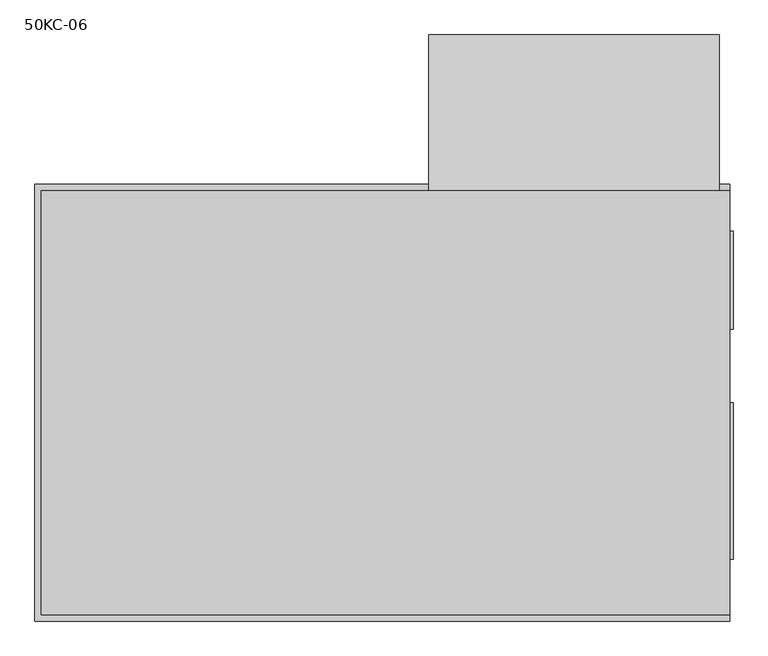
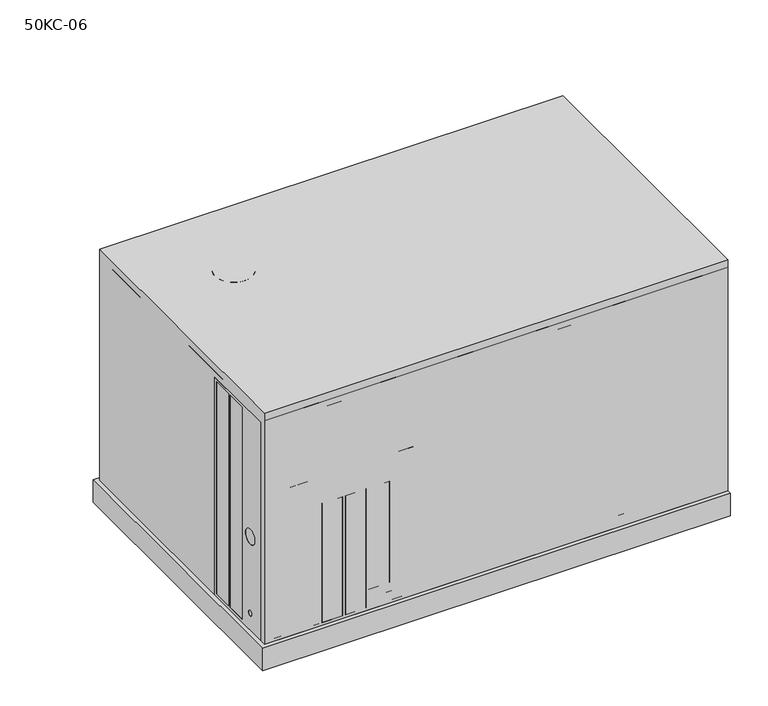
"""IFC4 building model written with IfcOpenShell, lengths in millimetres: proxy geometry, AHU-Rooftop-Carrier-Cooling_&_Elec_Heating-3-5_ton : 50KC-06."""

import ifcopenshell
import ifcopenshell.guid

model = None  # the IFC model being written
_history = None  # IfcOwnerHistory: only IFC2X3 demands one
_inside = {}  # id of a spatial element -> (the spatial element, [elements in it])
_under = {}  # id of a project, library or spatial element -> (it, [spatial elements below it])
_declared = {}  # id of a project -> (the project, [libraries it declares])
_typed = {}  # id of a type object -> (the type object, [elements of that type])
_made_of = {}  # id of a material, layer set ... -> (it, [elements and type objects made of it])


def new_model(schema):
    """Start an empty IFC model of exactly this schema.

    Asked for "IFC4X3", IfcOpenShell would pick the latest addendum, in which some entities
    have other attributes; the version numbers below select the first issue.
    IFC2X3 requires an IfcOwnerHistory on every rooted entity: one is made here for all.
    """
    global model, _history
    if schema == "IFC4X3":
        model = ifcopenshell.file(schema_version=(4, 3, 0, 0))
    else:
        model = ifcopenshell.file(schema=schema)
    _inside.clear()
    _under.clear()
    _declared.clear()
    _typed.clear()
    _made_of.clear()
    _history = None
    if model.schema == "IFC2X3":
        org = make("IfcOrganization", Name="unknown")
        user = make(
            "IfcPersonAndOrganization",
            ThePerson=make("IfcPerson", FamilyName="unknown"),
            TheOrganization=org,
        )
        app = make(
            "IfcApplication",
            ApplicationDeveloper=org,
            Version="unknown",
            ApplicationFullName="unknown",
            ApplicationIdentifier="unknown",
        )
        _history = make(
            "IfcOwnerHistory",
            OwningUser=user,
            OwningApplication=app,
            ChangeAction="ADDED",
            CreationDate=0,
        )
    return model


def make(cls, **values):
    """One entity of the class cls with the attributes given. An attribute that is None is left unset."""
    return model.create_entity(
        cls, **{name: value for name, value in values.items() if value is not None}
    )


def rooted(cls, **values):
    """An entity with a GlobalId (a new one), such as an element, a storey or a relation."""
    return make(cls, GlobalId=ifcopenshell.guid.new(), OwnerHistory=_history, **values)


def si_unit(unit_type, name, prefix=None):
    """IfcSIUnit, for example si_unit("LENGTHUNIT", "METRE", prefix="MILLI")."""
    return make("IfcSIUnit", UnitType=unit_type, Prefix=prefix, Name=name)


def assignment(units):
    """IfcUnitAssignment: the units of a project."""
    return None if units is None else make("IfcUnitAssignment", Units=units)


def point(xyz):
    """IfcCartesianPoint."""
    return None if xyz is None else make("IfcCartesianPoint", Coordinates=xyz)


def direction(xyz):
    """IfcDirection."""
    return None if xyz is None else make("IfcDirection", DirectionRatios=xyz)


def frame(location, z_axis=None, x_axis=None):
    """IfcAxis2Placement3D, a coordinate frame: its origin and axes. An axis left out is left unset."""
    return make(
        "IfcAxis2Placement3D",
        Location=point(location),
        Axis=direction(z_axis),
        RefDirection=direction(x_axis),
    )


def frame_2d(location, x_axis=None):
    """IfcAxis2Placement2D, a coordinate frame in the plane: its origin and x axis."""
    return make(
        "IfcAxis2Placement2D", Location=point(location), RefDirection=direction(x_axis)
    )


def origin():
    """The frame at (0, 0, 0) with its axes left unset."""
    return frame((0.0, 0.0, 0.0))


def origin_with_axes():
    """The frame at (0, 0, 0) with the z axis (0, 0, 1) and the x axis (1, 0, 0) written out."""
    return frame((0.0, 0.0, 0.0), z_axis=(0.0, 0.0, 1.0), x_axis=(1.0, 0.0, 0.0))


def place(relative_to, where):
    """IfcLocalPlacement: puts the frame where relative to a parent placement (None: the world)."""
    return make(
        "IfcLocalPlacement", PlacementRelTo=relative_to, RelativePlacement=where
    )


def context(
    kind, dimensions, precision=None, world=None, true_north=None, identifier=None
):
    """IfcGeometricRepresentationContext, for example the 3D "Model" context."""
    return make(
        "IfcGeometricRepresentationContext",
        ContextIdentifier=identifier,
        ContextType=kind,
        CoordinateSpaceDimension=dimensions,
        Precision=precision,
        WorldCoordinateSystem=world,
        TrueNorth=true_north,
    )


def project(units=None, contexts=None):
    """IfcProject with its units and contexts."""
    return rooted(
        "IfcProject",
        Name="project",
        RepresentationContexts=contexts,
        UnitsInContext=assignment(units),
    )


def spatial(cls, under=None, at=None, **own):
    """A site, building, storey or space (cls), placed at a placement, below another one or the project."""
    s = rooted(cls, ObjectPlacement=at, **own)
    if under is not None:
        _under.setdefault(under.id(), (under, []))[1].append(s)
    return s


def polyline(points):
    """IfcPolyline through the points."""
    return make("IfcPolyline", Points=[point(p) for p in points])


def circle_curve(where, radius):
    """IfcCircle in the frame where."""
    return make("IfcCircle", Position=where, Radius=radius)


def trimmed(basis, trim1, trim2, sense, master):
    """IfcTrimmedCurve: the piece of a basis curve between two trims."""
    return make(
        "IfcTrimmedCurve",
        BasisCurve=basis,
        Trim1=trim1,
        Trim2=trim2,
        SenseAgreement=sense,
        MasterRepresentation=master,
    )


def segment(curve, same_sense, transition):
    """IfcCompositeCurveSegment."""
    return make(
        "IfcCompositeCurveSegment",
        Transition=transition,
        SameSense=same_sense,
        ParentCurve=curve,
    )


def composite_curve(segments, self_intersect=None):
    """IfcCompositeCurve: segments joined end to end."""
    return make("IfcCompositeCurve", Segments=segments, SelfIntersect=self_intersect)


def outline(outer, holes=None, kind="AREA"):
    """IfcArbitraryClosedProfileDef: a profile drawn as a closed curve; with holes, ...WithVoids."""
    if holes is None:
        return make("IfcArbitraryClosedProfileDef", ProfileType=kind, OuterCurve=outer)
    return make(
        "IfcArbitraryProfileDefWithVoids",
        ProfileType=kind,
        OuterCurve=outer,
        InnerCurves=holes,
    )


def extrude(swept, where, along, depth):
    """IfcExtrudedAreaSolid: the profile swept, set in the frame where, extruded along a direction by depth."""
    return make(
        "IfcExtrudedAreaSolid",
        SweptArea=swept,
        Position=where,
        ExtrudedDirection=direction(along),
        Depth=depth,
    )


def faces_of(points, faces, orient=None, outer=None):
    """IfcFace entities. A face is a list of loops; a loop is a list of indices into points, from 0.

    orient and outer hold one flag for each loop. By default every Orientation is true, the
    first loop of a face is its IfcFaceOuterBound and the others are IfcFaceBound.
    """
    made = []
    for i, loops in enumerate(faces):
        bounds = []
        for j, loop in enumerate(loops):
            is_outer = j == 0 if outer is None else outer[i][j]
            bounds.append(
                make(
                    "IfcFaceOuterBound" if is_outer else "IfcFaceBound",
                    Bound=make("IfcPolyLoop", Polygon=[points[k] for k in loop]),
                    Orientation=True if orient is None else orient[i][j],
                )
            )
        made.append(make("IfcFace", Bounds=bounds))
    return made


def faceted_brep(points, faces, orient=None, outer=None, voids=None):
    """IfcFacetedBrep: a solid bounded by flat faces; with voids (closed shells), ...WithVoids."""
    shared = [point(p) for p in points]
    hull = make("IfcClosedShell", CfsFaces=faces_of(shared, faces, orient, outer))
    if voids is None:
        return make("IfcFacetedBrep", Outer=hull)
    return make(
        "IfcFacetedBrepWithVoids",
        Outer=hull,
        Voids=[
            make(cls, CfsFaces=faces_of(shared, fs, o, b)) for cls, fs, o, b in voids
        ],
    )


def shape(context_of_items, identifier, shape_type, items):
    """IfcShapeRepresentation: the items that make up one representation, for example the "Body"."""
    return make(
        "IfcShapeRepresentation",
        ContextOfItems=context_of_items,
        RepresentationIdentifier=identifier,
        RepresentationType=shape_type,
        Items=items,
    )


def source(mapping_origin, context_of_items, identifier, shape_type, items):
    """IfcRepresentationMap: a shape defined once, which mapped items show again and again."""
    return make(
        "IfcRepresentationMap",
        MappingOrigin=mapping_origin,
        MappedRepresentation=shape(context_of_items, identifier, shape_type, items),
    )


def transform(
    local_origin,
    x_axis=None,
    y_axis=None,
    z_axis=None,
    scale=None,
    scale2=None,
    scale3=None,
    uniform=True,
):
    """IfcCartesianTransformationOperator3D, or its non-uniform kind. x_axis, y_axis, z_axis: its Axis1, 2, 3."""
    if uniform:
        return make(
            "IfcCartesianTransformationOperator3D",
            Axis1=direction(x_axis),
            Axis2=direction(y_axis),
            LocalOrigin=point(local_origin),
            Scale=scale,
            Axis3=direction(z_axis),
        )
    return make(
        "IfcCartesianTransformationOperator3DnonUniform",
        Axis1=direction(x_axis),
        Axis2=direction(y_axis),
        LocalOrigin=point(local_origin),
        Scale=scale,
        Axis3=direction(z_axis),
        Scale2=scale2,
        Scale3=scale3,
    )


def mapped(mapping_source, mapping_target):
    """IfcMappedItem: shows the shape of a source again, moved by a transform."""
    return make(
        "IfcMappedItem", MappingSource=mapping_source, MappingTarget=mapping_target
    )


def made_of(thing, what):
    """Note that an element or type object is made of a material, layer set ...; save() writes the relation."""
    if what is not None:
        _made_of.setdefault(what.id(), (what, []))[1].append(thing)
    return thing


def element(
    cls,
    number,
    at=None,
    inside=None,
    cuts=None,
    type_object=None,
    material=None,
    context=None,
    identifier="Body",
    shape_type=None,
    held_by="IfcProductDefinitionShape",
    body=None,
    shapes=None,
    **own,
):
    """One element of the class cls, such as IfcWall. Its Tag is "e" and its number.

    at: its placement. inside: the storey or other place that contains it. cuts: it is an
    opening in that element (IfcRelVoidsElement). A single representation is given by context,
    identifier, shape_type and body (its items); several are given by shapes. held_by: the class
    of the entity that holds the representations. save() writes the other relations.
    """
    e = rooted(cls, Tag="e%d" % number, ObjectPlacement=at, **own)
    if body is not None:
        shapes = [shape(context, identifier, shape_type, body)]
    if shapes is not None:
        e.Representation = make(held_by, Representations=shapes)
    if inside is not None:
        _inside.setdefault(inside.id(), (inside, []))[1].append(e)
    if cuts is not None:
        rooted(
            "IfcRelVoidsElement", RelatingBuildingElement=cuts, RelatedOpeningElement=e
        )
    if type_object is not None:
        _typed.setdefault(type_object.id(), (type_object, []))[1].append(e)
    return made_of(e, material)


def aggregate(whole, parts):
    """IfcRelAggregates: a whole, such as a stair, and the parts it consists of."""
    return rooted("IfcRelAggregates", RelatingObject=whole, RelatedObjects=parts)


def save(model, path):
    """Write the relations noted so far, then the file.

    IfcRelAggregates (storeys below a building ...), IfcRelContainedInSpatialStructure (elements
    in a storey), IfcRelDefinesByType, IfcRelAssociatesMaterial and IfcRelDeclares: one each for
    every whole, place, type object, material and project.
    """
    for whole, parts in _under.values():
        aggregate(whole, parts)
    for where, things in _inside.values():
        rooted(
            "IfcRelContainedInSpatialStructure",
            RelatedElements=things,
            RelatingStructure=where,
        )
    for kind, things in _typed.values():
        rooted("IfcRelDefinesByType", RelatedObjects=things, RelatingType=kind)
    for what, things in _made_of.values():
        rooted("IfcRelAssociatesMaterial", RelatedObjects=things, RelatingMaterial=what)
    for by, libraries in _declared.values():
        rooted("IfcRelDeclares", RelatingContext=by, RelatedDefinitions=libraries)
    model.write(path)


def plane_surface(at):
    """IfcPlane: the flat surface through the origin of the frame at, square to its z axis."""
    return make("IfcPlane", Position=at)


def cylinder_surface(at, radius):
    """IfcCylindricalSurface: all points at the distance radius from the z axis of the frame at."""
    return make("IfcCylindricalSurface", Position=at, Radius=radius)


def revolved_surface(curve, axis_point, axis_direction):
    """IfcSurfaceOfRevolution: the curve turned about the line through axis_point along axis_direction."""
    return make(
        "IfcSurfaceOfRevolution",
        SweptCurve=make("IfcArbitraryOpenProfileDef", ProfileType="CURVE", Curve=curve),
        AxisPosition=make("IfcAxis1Placement", Location=point(axis_point), Axis=direction(axis_direction)),
    )


def advanced_brep(points, edges, surfaces, faces):
    """IfcAdvancedBrep: a solid bounded by faces that lie on surfaces and meet in shared edges.

    An edge is (start, end): straight between two places in points (the first is 0);
    or (start, end, curve); or (start, end, curve, False) where it runs against its curve.
    A face is (place in surfaces, loops), or (place, loops, False) where it looks against
    its surface's normal. A loop lists edges by number (the first is 1), with a minus sign
    where the edge is run from its end to its start. The first loop is the outer one.
    """
    corners = [point(p) for p in points]
    vertices = [make("IfcVertexPoint", VertexGeometry=c) for c in corners]
    made = []
    for start, end, *more in edges:
        made.append(
            make(
                "IfcEdgeCurve",
                EdgeStart=vertices[start],
                EdgeEnd=vertices[end],
                EdgeGeometry=more[0] if more else make("IfcPolyline", Points=[corners[start], corners[end]]),
                SameSense=more[1] if len(more) > 1 else True,
            )
        )
    hull = []
    for where, loops, *sense in faces:
        bounds = []
        for j, loop in enumerate(loops):
            ring = [make("IfcOrientedEdge", EdgeElement=made[abs(k) - 1], Orientation=k > 0) for k in loop]
            bounds.append(
                make(
                    "IfcFaceOuterBound" if j == 0 else "IfcFaceBound",
                    Bound=make("IfcEdgeLoop", EdgeList=ring),
                    Orientation=True,
                )
            )
        hull.append(make("IfcAdvancedFace", Bounds=bounds, FaceSurface=surfaces[where], SameSense=sense[0] if sense else True))
    return make("IfcAdvancedBrep", Outer=make("IfcClosedShell", CfsFaces=hull))


def proxy_50kc_06_755dc8fb(model_context):
    return source(origin(), model_context, "Body", "SolidModel", [
        extrude(outline(polyline([(-547.6875, 1025.525), (-228.6, 1025.525), (-228.6, 95.25), (-547.6875, 95.25), (-547.6875, 1025.525)]), holes=[polyline([(-323.85, 1012.825), (-323.85, 107.95), (-241.3, 107.95), (-241.3, 1012.825), (-323.85, 1012.825)]), polyline([(-419.1, 1012.825), (-419.1, 107.95), (-336.55, 107.95), (-336.55, 1012.825), (-419.1, 1012.825)]), composite_curve([segment(trimmed(circle_curve(frame_2d((-476.25, 495.3)), 31.75), [point((-508.0, 495.3))], [point((-444.5, 495.3))], True, "CARTESIAN"), True, "CONTINUOUS"), segment(trimmed(circle_curve(frame_2d((-476.25, 495.3)), 31.75), [point((-444.5, 495.3))], [point((-508.0, 495.3))], True, "CARTESIAN"), True, "CONTINUOUS")], self_intersect=False), composite_curve([segment(trimmed(circle_curve(frame_2d((-476.25, 168.275)), 11.1125), [point((-487.3625, 168.275))], [point((-465.1375, 168.275))], True, "CARTESIAN"), True, "CONTINUOUS"), segment(trimmed(circle_curve(frame_2d((-476.25, 168.275)), 11.1125), [point((-465.1375, 168.275))], [point((-487.3625, 168.275))], True, "CARTESIAN"), True, "CONTINUOUS")], self_intersect=False)]), frame((-927.1, 0.0, 0.0), z_axis=(1.0, 0.0, 0.0), x_axis=(0.0, 1.0, 0.0)), (0.0, 0.0, 1.0), 3.175),
        advanced_brep(
        [(941.3875, 573.0875, 1025.525), (-436.5625, 573.0875, 1025.525), (-436.5625, 534.9875, 1025.525), (-885.825, 534.9875, 1025.525), (-885.825, -215.9, 1025.525), (-923.925, -215.9, 1025.525), (-923.925, -573.0875, 1025.525), (941.3875, -573.0875, 1025.525), (-883.285, 532.4475, 1025.525), (-436.5625, 532.4475, 1025.525), (-436.5625, -215.9, 1025.525), (-883.285, -215.9, 1025.525), (941.3875, 573.0875, 95.25), (941.3875, -573.0875, 95.25), (-923.925, -573.0875, 95.25), (-923.925, -215.9, 95.25), (-885.825, -215.9, 95.25), (-885.825, 534.9875, 95.25), (-436.5625, 534.9875, 95.25), (-436.5625, 573.0875, 95.25), (-883.285, 532.4475, 95.25), (-883.285, -215.9, 95.25), (-436.5625, -215.9, 95.25), (-436.5625, 532.4475, 95.25), (-923.925, -508.0, 495.3), (-923.925, -444.5, 495.3), (-923.925, -487.3625, 168.275), (-923.925, -465.1375, 168.275), (941.3875, 88.9, 194.1909375), (941.3875, 88.9, 161.4090625), (919.1625, 88.9, 161.4090625), (919.1625, 88.9, 194.1909375), (-914.4, -508.0, 495.3), (-914.4, -444.5, 495.3), (-914.4, -487.3625, 168.275), (-914.4, -465.1375, 168.275)],
        [
            (0, 1),
            (1, 2),
            (2, 3),
            (3, 4),
            (4, 5),
            (5, 6),
            (6, 7),
            (7, 0),
            (8, 9),
            (9, 10),
            (10, 11),
            (11, 8),
            (12, 13),
            (13, 14),
            (14, 15),
            (15, 16),
            (16, 17),
            (17, 18),
            (18, 19),
            (19, 12),
            (20, 21),
            (21, 22),
            (22, 23),
            (23, 20),
            (0, 12),
            (19, 1),
            (5, 15),
            (14, 6),
            (24, 25, circle_curve(frame((-923.925, -476.25, 495.3), z_axis=(1.0, 0.0, 0.0), x_axis=(0.0, 1.0, 0.0)), 31.75)),
            (25, 24, circle_curve(frame((-923.925, -476.25, 495.3), z_axis=(1.0, 0.0, 0.0), x_axis=(0.0, 1.0, 0.0)), 31.75)),
            (26, 27, circle_curve(frame((-923.925, -476.25, 168.275), z_axis=(1.0, 0.0, 0.0), x_axis=(0.0, 1.0, 0.0)), 11.1125)),
            (27, 26, circle_curve(frame((-923.925, -476.25, 168.275), z_axis=(1.0, 0.0, 0.0), x_axis=(0.0, 1.0, 0.0)), 11.1125)),
            (13, 7),
            (28, 29, circle_curve(frame((941.3875, 88.9, 177.8), z_axis=(-1.0, 0.0, 0.0), x_axis=(0.0, 0.0, 1.0)), 16.3909375)),
            (29, 28, circle_curve(frame((941.3875, 88.9, 177.8), z_axis=(-1.0, 0.0, 0.0), x_axis=(0.0, 0.0, 1.0)), 16.3909375)),
            (18, 2),
            (17, 3),
            (16, 4),
            (30, 31, circle_curve(frame((919.1625, 88.9, 177.8), z_axis=(1.0, 0.0, 0.0), x_axis=(0.0, 0.0, 1.0)), 16.3909375)),
            (31, 30, circle_curve(frame((919.1625, 88.9, 177.8), z_axis=(1.0, 0.0, 0.0), x_axis=(0.0, 0.0, 1.0)), 16.3909375)),
            (30, 29),
            (28, 31),
            (32, 33, circle_curve(frame((-914.4, -476.25, 495.3), z_axis=(-1.0, 0.0, 0.0), x_axis=(0.0, 1.0, 0.0)), 31.75)),
            (33, 32, circle_curve(frame((-914.4, -476.25, 495.3), z_axis=(-1.0, 0.0, 0.0), x_axis=(0.0, 1.0, 0.0)), 31.75)),
            (34, 35, circle_curve(frame((-914.4, -476.25, 168.275), z_axis=(-1.0, 0.0, 0.0), x_axis=(0.0, 1.0, 0.0)), 11.1125)),
            (35, 34, circle_curve(frame((-914.4, -476.25, 168.275), z_axis=(-1.0, 0.0, 0.0), x_axis=(0.0, 1.0, 0.0)), 11.1125)),
            (33, 25),
            (24, 32),
            (35, 27),
            (26, 34),
            (8, 20),
            (23, 9),
            (22, 10),
            (21, 11),
        ],
        [
            plane_surface(frame((-466.3462048, 573.0875, 1025.525), z_axis=(0.0, 0.0, 1.0), x_axis=(-1.0, 0.0, 0.0))),
            plane_surface(frame((-466.3462048, 573.0875, 95.25), z_axis=(0.0, 0.0, -1.0), x_axis=(1.0, 0.0, 0.0))),
            plane_surface(frame((941.3875, 573.0875, 1025.525), z_axis=(0.0, 1.0, 0.0), x_axis=(0.0, 0.0, -1.0))),
            plane_surface(frame((-923.925, -215.9, 1025.525), z_axis=(-1.0, 0.0, 0.0), x_axis=(0.0, 0.0, -1.0))),
            plane_surface(frame((-923.925, -573.0875, 1025.525), z_axis=(0.0, -1.0, 0.0), x_axis=(0.0, 0.0, -1.0))),
            plane_surface(frame((941.3875, -573.0875, 1025.525), z_axis=(1.0, 0.0, 0.0), x_axis=(0.0, 0.0, -1.0))),
            plane_surface(frame((-436.5625, 573.0875, 1025.525), z_axis=(-1.0, 0.0, 0.0), x_axis=(0.0, 0.0, -1.0))),
            plane_surface(frame((-436.5625, 534.9875, 1025.525), z_axis=(0.0, 1.0, 0.0), x_axis=(0.0, 0.0, -1.0))),
            plane_surface(frame((-885.825, 534.9875, 1025.525), z_axis=(-1.0, 0.0, 0.0), x_axis=(0.0, 0.0, -1.0))),
            plane_surface(frame((-885.825, -215.9, 1025.525), z_axis=(0.0, 1.0, 0.0), x_axis=(0.0, 0.0, -1.0))),
            plane_surface(frame((919.1625, 88.9, 177.8), z_axis=(1.0, 0.0, 0.0), x_axis=(0.0, 1.0, 0.0))),
            revolved_surface(polyline([(941.3875, 88.9, 194.19093750000002), (919.1625, 88.9, 194.19093750000002)]), (944.5625, 88.9, 177.8), (1.0, 0.0, 0.0)),
            plane_surface(frame((-914.4, -444.5, 495.3), z_axis=(-1.0, 0.0, 0.0), x_axis=(0.0, 0.0, 1.0))),
            revolved_surface(polyline([(-914.4, -444.5, 495.3), (-923.925, -444.5, 495.3)]), (-927.1, -476.25, 495.3), (1.0, 0.0, 0.0)),
            revolved_surface(polyline([(-914.4, -465.1375, 168.275), (-923.925, -465.1375, 168.275)]), (-927.1, -476.25, 168.275), (1.0, 0.0, 0.0)),
            plane_surface(frame((-883.285, 532.4475, 1025.525), z_axis=(0.0, -1.0, 0.0), x_axis=(0.0, 0.0, -1.0))),
            plane_surface(frame((-436.5625, 532.4475, 1025.525), z_axis=(-1.0, 0.0, 0.0), x_axis=(0.0, 0.0, -1.0))),
            plane_surface(frame((-436.5625, -215.9, 1025.525), z_axis=(0.0, 1.0, 0.0), x_axis=(0.0, 0.0, -1.0))),
            plane_surface(frame((-883.285, -215.9, 1025.525), z_axis=(1.0, 0.0, 0.0), x_axis=(0.0, 0.0, -1.0))),
        ],
        [
            (0, [[1, 2, 3, 4, 5, 6, 7, 8], [9, 10, 11, 12]]),
            (1, [[13, 14, 15, 16, 17, 18, 19, 20], [21, 22, 23, 24]]),
            (2, [[-1, 25, -20, 26]]),
            (3, [[-6, 27, -15, 28], [29, 30], [31, 32]]),
            (4, [[-7, -28, -14, 33]]),
            (5, [[-8, -33, -13, -25], [34, 35]]),
            (6, [[-2, -26, -19, 36]]),
            (7, [[-3, -36, -18, 37]]),
            (8, [[-4, -37, -17, 38]]),
            (9, [[-5, -38, -16, -27]]),
            (10, [[39, 40]]),
            (11, [[-39, 41, -34, 42]]),
            (11, [[-40, -42, -35, -41]]),
            (12, [[43, 44]]),
            (12, [[45, 46]]),
            (13, [[-44, 47, -29, 48]]),
            (13, [[-43, -48, -30, -47]]),
            (14, [[-46, 49, -31, 50]]),
            (14, [[-45, -50, -32, -49]]),
            (15, [[-9, 51, -24, 52]]),
            (16, [[-10, -52, -23, 53]]),
            (17, [[-11, -53, -22, 54]]),
            (18, [[-12, -54, -21, -51]]),
        ],
    ),
        faceted_brep([(-898.525, 573.0875, 1025.525), (-923.925, 573.0875, 1025.525), (-923.925, 547.6875, 1025.525), (-898.525, 547.6875, 1025.525), (-898.525, 573.0875, 95.25), (-898.525, 547.6875, 95.25), (-923.925, 547.6875, 95.25), (-923.925, 573.0875, 95.25)], [[[0, 1, 2, 3]], [[4, 5, 6, 7]], [[1, 0, 4, 7]], [[2, 1, 7, 6]], [[3, 2, 6, 5]], [[0, 3, 5, 4]]]),
        extrude(outline(polyline([(941.3875, 466.725), (954.0875, 466.725), (954.0875, 200.025), (941.3875, 200.025), (941.3875, 466.725)])), frame((0.0, 0.0, 155.575), z_axis=(0.0, 0.0, 1.0), x_axis=(1.0, 0.0, 0.0)), (0.0, 0.0, 1.0), 638.175),
        extrude(outline(polyline([(941.3875, 0.0), (954.0875, 0.0), (954.0875, -425.45), (941.3875, -425.45), (941.3875, 0.0)])), frame((0.0, 0.0, 155.575), z_axis=(0.0, 0.0, 1.0), x_axis=(1.0, 0.0, 0.0)), (0.0, 0.0, 1.0), 288.925),
        extrude(outline(polyline([(944.5625, 576.2625), (944.5625, -576.2625), (-927.1, -576.2625), (-927.1, 576.2625), (944.5625, 576.2625)])), frame((0.0, 0.0, 95.25), z_axis=(0.0, 0.0, 1.0), x_axis=(1.0, 0.0, 0.0)), (0.0, 0.0, 1.0), 987.425),
        extrude(outline(polyline([(-944.5625, 593.725), (944.5625, 593.725), (944.5625, -593.725), (-944.5625, -593.725), (-944.5625, 593.725)])), origin_with_axes(), (0.0, 0.0, 1.0), 95.25),
        extrude(outline(polyline([(21.43125, -576.2625), (-3.96875, -576.2625), (-3.96875, 576.2625), (21.43125, 576.2625), (21.43125, -576.2625)])), frame((0.0, 0.0, 1050.925), z_axis=(0.0, 0.0, 1.0), x_axis=(1.0, 0.0, 0.0)), (0.0, 0.0, 1.0), 12.7),
        extrude(outline(polyline([(1025.525, -411.1625), (95.25, -411.1625), (95.25, 101.6), (1025.525, 101.6), (1025.525, -411.1625)]), holes=[polyline([(177.8, -202.40625), (177.8, -107.15625), (146.05, -107.15625), (146.05, -202.40625), (177.8, -202.40625)])]), frame((0.0, 573.0875, 0.0), z_axis=(0.0, 1.0, 0.0), x_axis=(0.0, 0.0, 1.0)), (0.0, 0.0, 1.0), 3.175),
        extrude(outline(polyline([(915.9875, 573.0875), (127.0, 573.0875), (127.0, 576.2625), (915.9875, 576.2625), (915.9875, 573.0875)])), frame((0.0, 0.0, 546.1), z_axis=(0.0, 0.0, 1.0), x_axis=(1.0, 0.0, 0.0)), (0.0, 0.0, 1.0), 479.425),
        extrude(outline(polyline([(915.9875, 573.0875), (127.0, 573.0875), (127.0, 576.2625), (915.9875, 576.2625), (915.9875, 573.0875)])), frame((0.0, 0.0, 95.25), z_axis=(0.0, 0.0, 1.0), x_axis=(1.0, 0.0, 0.0)), (0.0, 0.0, 1.0), 444.5),
        extrude(outline(polyline([(-923.925, -336.55), (-923.925, -419.1), (-927.1, -419.1), (-927.1, -336.55), (-923.925, -336.55)])), frame((0.0, 0.0, 107.95), z_axis=(0.0, 0.0, 1.0), x_axis=(1.0, 0.0, 0.0)), (0.0, 0.0, 1.0), 904.875),
        extrude(outline(polyline([(-923.925, -241.3), (-923.925, -323.85), (-927.1, -323.85), (-927.1, -241.3), (-923.925, -241.3)])), frame((0.0, 0.0, 107.95), z_axis=(0.0, 0.0, 1.0), x_axis=(1.0, 0.0, 0.0)), (0.0, 0.0, 1.0), 904.875),
        extrude(outline(polyline([(-803.275, -576.2625), (-885.825, -576.2625), (-885.825, -573.0875), (-803.275, -573.0875), (-803.275, -576.2625)])), frame((0.0, 0.0, 107.95), z_axis=(0.0, 0.0, 1.0), x_axis=(1.0, 0.0, 0.0)), (0.0, 0.0, 1.0), 622.3),
        extrude(outline(polyline([(-708.025, -576.2625), (-790.575, -576.2625), (-790.575, -573.0875), (-708.025, -573.0875), (-708.025, -576.2625)])), frame((0.0, 0.0, 107.95), z_axis=(0.0, 0.0, 1.0), x_axis=(1.0, 0.0, 0.0)), (0.0, 0.0, 1.0), 622.3),
        extrude(outline(polyline([(-612.775, -576.2625), (-695.325, -576.2625), (-695.325, -573.0875), (-612.775, -573.0875), (-612.775, -576.2625)])), frame((0.0, 0.0, 107.95), z_axis=(0.0, 0.0, 1.0), x_axis=(1.0, 0.0, 0.0)), (0.0, 0.0, 1.0), 508.0),
        extrude(outline(polyline([(-517.525, -576.2625), (-600.075, -576.2625), (-600.075, -573.0875), (-517.525, -573.0875), (-517.525, -576.2625)])), frame((0.0, 0.0, 107.95), z_axis=(0.0, 0.0, 1.0), x_axis=(1.0, 0.0, 0.0)), (0.0, 0.0, 1.0), 508.0),
        extrude(outline(polyline([(-422.275, -576.2625), (-504.825, -576.2625), (-504.825, -573.0875), (-422.275, -573.0875), (-422.275, -576.2625)])), frame((0.0, 0.0, 184.15), z_axis=(0.0, 0.0, 1.0), x_axis=(1.0, 0.0, 0.0)), (0.0, 0.0, 1.0), 431.8),
        extrude(outline(polyline([(-327.025, -576.2625), (-409.575, -576.2625), (-409.575, -573.0875), (-327.025, -573.0875), (-327.025, -576.2625)])), frame((0.0, 0.0, 107.95), z_axis=(0.0, 0.0, 1.0), x_axis=(1.0, 0.0, 0.0)), (0.0, 0.0, 1.0), 622.3),
        extrude(outline(polyline([(1025.525, 915.9875), (1025.525, 34.13125), (95.25, 34.13125), (95.25, 915.9875), (1025.525, 915.9875)]), holes=[polyline([(177.8, 522.684375), (146.05, 522.684375), (146.05, 427.434375), (177.8, 427.434375), (177.8, 522.684375)])]), frame((0.0, -576.2625, 0.0), z_axis=(0.0, 1.0, 0.0), x_axis=(0.0, 0.0, 1.0)), (0.0, 0.0, 1.0), 3.175),
        extrude(outline(polyline([(1025.525, -16.66875), (1025.525, -898.525), (95.25, -898.525), (95.25, -16.66875), (1025.525, -16.66875)]), holes=[polyline([(177.8, -415.925), (146.05, -415.925), (146.05, -511.175), (177.8, -511.175), (177.8, -415.925)]), polyline([(730.25, -803.275), (107.95, -803.275), (107.95, -885.825), (730.25, -885.825), (730.25, -803.275)]), polyline([(730.25, -708.025), (107.95, -708.025), (107.95, -790.575), (730.25, -790.575), (730.25, -708.025)]), polyline([(615.95, -612.775), (107.95, -612.775), (107.95, -695.325), (615.95, -695.325), (615.95, -612.775)]), polyline([(615.95, -517.525), (107.95, -517.525), (107.95, -600.075), (615.95, -600.075), (615.95, -517.525)]), polyline([(615.95, -422.275), (184.15, -422.275), (184.15, -504.825), (615.95, -504.825), (615.95, -422.275)]), polyline([(730.25, -327.025), (107.95, -327.025), (107.95, -409.575), (730.25, -409.575), (730.25, -327.025)])]), frame((0.0, -576.2625, 0.0), z_axis=(0.0, 1.0, 0.0), x_axis=(0.0, 0.0, 1.0)), (0.0, 0.0, 1.0), 3.175),
        extrude(outline(polyline([(1000.125, 464.451767), (997.9196681, 451.9447085), (947.8914343, 460.7660359), (709.1843069, 119.8569277), (573.0875, 107.95), (573.0875, 539.75), (1000.125, 464.451767)])), frame((127.0, 0.0, 0.0), z_axis=(1.0, 0.0, 0.0), x_axis=(0.0, 1.0, 0.0)), (0.0, 0.0, 1.0), 788.9875),
        advanced_brep(
        [(-584.2, 233.3625, 1082.675), (-660.4, 233.3625, 1082.675), (-508.0, 233.3625, 1082.675), (-660.4, 233.3625, 1079.5), (-508.0, 233.3625, 1079.5), (-863.6, 233.3625, 1050.925), (-304.8, 233.3625, 1050.925), (-584.2, 233.3625, 1050.925)],
        [
            (0, 1),
            (1, 2, circle_curve(frame((-584.2, 233.3625, 1082.675), z_axis=(0.0, 0.0, 1.0), x_axis=(-1.0, 0.0, 0.0)), 76.2)),
            (2, 0),
            (2, 1, circle_curve(frame((-584.2, 233.3625, 1082.675), z_axis=(0.0, 0.0, 1.0), x_axis=(-1.0, 0.0, 0.0)), 76.2)),
            (1, 3),
            (3, 4, circle_curve(frame((-584.2, 233.3625, 1079.5), z_axis=(0.0, 0.0, 1.0), x_axis=(-1.0, 0.0, 0.0)), 76.2)),
            (4, 2),
            (4, 3, circle_curve(frame((-584.2, 233.3625, 1079.5), z_axis=(0.0, 0.0, 1.0), x_axis=(-1.0, 0.0, 0.0)), 76.2)),
            (3, 5),
            (5, 6, circle_curve(frame((-584.2, 233.3625, 1050.925), z_axis=(0.0, 0.0, 1.0), x_axis=(-1.0, 0.0, 0.0)), 279.4)),
            (6, 4),
            (6, 5, circle_curve(frame((-584.2, 233.3625, 1050.925), z_axis=(0.0, 0.0, 1.0), x_axis=(-1.0, 0.0, 0.0)), 279.4)),
            (5, 7),
            (7, 6),
        ],
        [
            plane_surface(frame((-584.2, 233.3625, 1082.675), z_axis=(0.0, 0.0, 1.0), x_axis=(-1.0, 0.0, 0.0))),
            cylinder_surface(frame((-584.2, 233.3625, 1654.166912), z_axis=(0.0, 0.0, 1.0), x_axis=(-1.0, 0.0, 0.0)), 76.2),
            revolved_surface(polyline([(-863.6, 233.3625, 1050.925), (-660.4, 233.3625, 1079.5)]), (-584.2, 233.3625, 1654.166912), (0.0, 0.0, 1.0)),
            plane_surface(frame((-584.2, 233.3625, 1050.925), z_axis=(0.0, 0.0, -1.0), x_axis=(-1.0, 0.0, 0.0))),
        ],
        [
            (0, [[1, 2, 3]]),
            (0, [[-3, 4, -1]]),
            (1, [[-2, 5, 6, 7]]),
            (1, [[-4, -7, 8, -5]]),
            (2, [[-6, 9, 10, 11]]),
            (2, [[-8, -11, 12, -9]]),
            (3, [[-10, 13, 14]]),
            (3, [[-12, -14, -13]]),
        ],
    ),
        extrude(outline(polyline([(944.5625, 576.2625), (944.5625, -576.2625), (-927.1, -576.2625), (-927.1, 576.2625), (944.5625, 576.2625)])), frame((0.0, 0.0, 1025.525), z_axis=(0.0, 0.0, 1.0), x_axis=(1.0, 0.0, 0.0)), (0.0, 0.0, 1.0), 25.4),
        extrude(outline(polyline([(944.5625, 593.725), (944.5625, -593.725), (-944.5625, -593.725), (-944.5625, 593.725), (944.5625, 593.725)]), holes=[polyline([(877.8875, 527.05), (-877.8875, 527.05), (-877.8875, -527.05), (877.8875, -527.05), (877.8875, 527.05)])]), origin_with_axes(), (0.0, 0.0, 1.0), 95.25),
    ])


if __name__ == "__main__":
    model = new_model("IFC4")
    model_context = context("Model", 3, world=origin())
    ifc_project = project(units=[si_unit("LENGTHUNIT", "METRE", prefix="MILLI")], contexts=[model_context])
    site = spatial("IfcSite", under=ifc_project)
    building = spatial("IfcBuilding", under=site)
    placement = place(None, origin())
    proxy_50kc_06_shape = proxy_50kc_06_755dc8fb(model_context)
    element("IfcBuildingElementProxy", 1, Name="AHU-Rooftop-Carrier-Cooling_&_Elec_Heating-3-5_ton : 50KC-06", ObjectType="AHU-Rooftop-Carrier-Cooling_&_Elec_Heating-3-5_ton : 50KC-06", at=placement, inside=building, context=model_context, shape_type="MappedRepresentation", body=[
        mapped(proxy_50kc_06_shape, transform((0.0, 0.0, 0.0), x_axis=(1.0, 0.0, 0.0), y_axis=(0.0, 1.0, 0.0), z_axis=(0.0, 0.0, 1.0))),
    ])
    save(model, "model.ifc")

# Revit data of these elements
# Type "AHU-Rooftop-Carrier-Cooling_&_Elec_Heating-3-5_ton : 50KC-06"
#   URL = "www.carrier.com"
#   Model = "50KC-06"
#   Manufacturer = "Carrier Corporation"
#   Assembly Code = "D3050200"
#   Width = 3' - 10 3/4"
#   Voltage [instance default] = 240 V
#   SA Z Offset [instance default] = 0' - 2 3/8"
#   SA Y Offset [instance default] = 0' - 6 5/8"
#   SA X Offset [instance default] = 0' - 0"
#   SA Width [instance default] = 16 3/4"
#   SA Height [instance default] = 11 3/8"
#   RA Z Offset [instance default] = 0' - 2 3/8"
#   RA Y Offset [instance default] = 2' - 7 1/4"
#   RA X Offset [instance default] = 0' - 0"
#   RA Width [instance default] = 10 1/2"
#   RA Height [instance default] = 25 1/8"
#   Power Factor [instance default] = 0.8
#   Lid Lap = 0' - 0 1/8"
#   Lid Height = 0' - 1"
#   Length 9 [instance default] = 0' - 0"
#   Length 8 [instance default] = 0' - 0"
#   Length 7 [instance default] = 0' - 0"
#   Length 6 [instance default] = 0' - 0"
#   Length 5 [instance default] = 0' - 0"
#   Length 4 = 0' - 1"
#   Length 3 [instance default] = 1' - 4"
#   Length 2 = 1' - 1 1/2"
#   Length 1 [instance default] = 0' - 0"
#   Length = 6' - 2 3/8"
#   Height = 3' - 5 3/8"
#   Handle Width = 0' - 3 3/4"
#   Handle Height = 0' - 1 1/4"
#   Grille Radius = 0' - 11"
#   Grille Plate Radius = 0' - 3"
#   Frame Width = 0' - 1"
#   Fan Height = 0' - 1 1/4"
#   Electrical Panel Length = 1' - 2 7/8"
#   Economizer Width = 1' - 4"
#   Economizer Offset = 1' - 9 1/4"
#   Economizer Length = 2' - 7 1/16"
#   Economizer Height = 1' - 5"
#   Drain Z Offset [instance default] = 0' - 3 1/4"
#   Drain Y Offset [instance default] = 2' - 2 7/8"
#   Drain X Offset [instance default] = 0' - 0"
#   Drain Radius [instance default] = 3/8"
#   Drain Hole Radius [instance default] = 0' - 0.64531"
#   Curb Width = 0' - 2 5/8"
#   Curb Height = 0' - 3 3/4"
#   Clearance Top [instance default] = 5' - 0"
#   Clearance Right [instance default] = 3' - 0"
#   Clearance Left [instance default] = 4' - 0"
#   Clearance Front [instance default] = 4' - 0"
#   Clearance Back [instance default] = 3' - 6"
#   Apparent Load [instance default] = 0 VA
#   Angle 3 [instance default] = 270.00°
#   Angle 2 [instance default] = 90.00°
#   Angle 1 [instance default] = 90.00°
#   Vertical Supply Air [instance default] = no
#   Vertical Return Air [instance default] = no
#   Standard Drain [instance default] = yes
#   Roof Curb [instance default] = yes
#   Number of Poles [instance default] = 3
#   Horizontal Supply Air [instance default] = yes
#   Horizontal Return Air [instance default] = yes
#   Economizer [instance default] = yes
#   Clearance Zones [instance default] = no
#   Alternate Drain [instance default] = no
#   Load Classification = HVAC
#   Highlight Material = Paint - Carrier - Black
#   Grille Material = Metal - Carrier - Grille 2
#   Fan Material = Metal - Carrier - Grille
#   Curb Material = Metal - Carrier - Steel
#   Clearance Material = Clearance Zone
#   Body Material = RTU PLACEHOLDER - SIZE TBD
# Element 1 (IfcBuildingElementProxy, "AHU-Rooftop-Carrier-Cooling_&_Elec_Heating-3-5_ton : 50KC-06")
#   Materials on its faces: "RTU PLACEHOLDER - SIZE TBD", "Metal - Carrier - Grille 2", "Metal - Carrier - Steel", "Paint - Carrier - Black", "Metal - Carrier - Grille"
# Materials
#   "Paint - Carrier - Black": class "Miscellaneous", colour RGB 46 46 46, transparency 0
#   "Metal - Carrier - Grille 2": class "Miscellaneous", colour RGB 182 199 209, transparency 0
#   "Metal - Carrier - Grille": class "Miscellaneous", colour RGB 115 113 111, transparency 0
#   "Metal - Carrier - Steel": class "Miscellaneous", colour RGB 192 192 192, transparency 0
#   "Clearance Zone": class "Glass", colour RGB 255 0 0, transparency 0.85
#   "RTU PLACEHOLDER - SIZE TBD": class "Miscellaneous", colour RGB 182 199 209, transparency 0, Cost = 0
